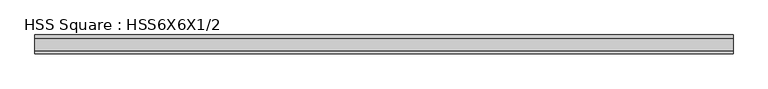
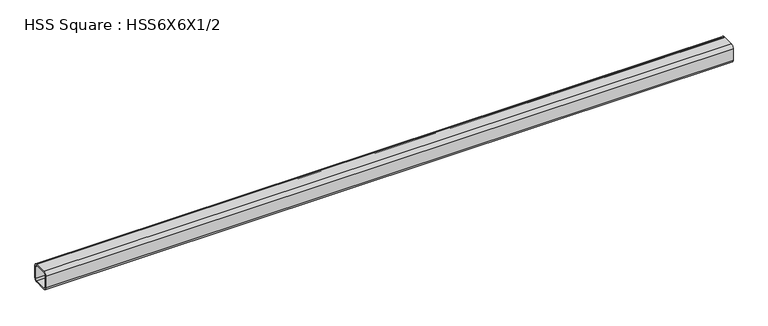
"""IFC4 building model written with IfcOpenShell, lengths in millimetres: member geometry, HSS Square : HSS6X6X1/2."""

from ifc_helpers import new_model, si_unit, point, frame, frame_2d, origin, place, context, project, spatial, polyline, circle_curve, trimmed, segment, composite_curve, outline, extrude, source, transform, mapped, element, save


def hss_square_hss6x6x1_2_6b3df641(model_context):
    return source(origin(), model_context, "Body", "SweptSolid", [
        extrude(outline(composite_curve([segment(polyline([(76.2, 50.8), (76.2, -50.8)]), True, "CONTINUOUS"), segment(trimmed(circle_curve(frame_2d((50.8, -50.8)), 25.4), [point((76.2, -50.8))], [point((50.8, -76.2))], False, "CARTESIAN"), True, "CONTINUOUS"), segment(polyline([(50.8, -76.2), (-50.8, -76.2)]), True, "CONTINUOUS"), segment(trimmed(circle_curve(frame_2d((-50.8, -50.8)), 25.4), [point((-50.8, -76.2))], [point((-76.2, -50.8))], False, "CARTESIAN"), True, "CONTINUOUS"), segment(polyline([(-76.2, -50.8), (-76.2, 50.8)]), True, "CONTINUOUS"), segment(trimmed(circle_curve(frame_2d((-50.8, 50.8)), 25.4), [point((-76.2, 50.8))], [point((-50.8, 76.2))], False, "CARTESIAN"), True, "CONTINUOUS"), segment(polyline([(-50.8, 76.2), (50.8, 76.2)]), True, "CONTINUOUS"), segment(trimmed(circle_curve(frame_2d((50.8, 50.8)), 25.4), [point((50.8, 76.2))], [point((76.2, 50.8))], False, "CARTESIAN"), True, "CONTINUOUS")], self_intersect=False), holes=[composite_curve([segment(trimmed(circle_curve(frame_2d((-50.8, 50.8)), 12.7), [point((-50.8, 63.5))], [point((-63.5, 50.8))], True, "CARTESIAN"), True, "CONTINUOUS"), segment(polyline([(-63.5, 50.8), (-63.5, -50.8)]), True, "CONTINUOUS"), segment(trimmed(circle_curve(frame_2d((-50.8, -50.8)), 12.7), [point((-63.5, -50.8))], [point((-50.8, -63.5))], True, "CARTESIAN"), True, "CONTINUOUS"), segment(polyline([(-50.8, -63.5), (50.8, -63.5)]), True, "CONTINUOUS"), segment(trimmed(circle_curve(frame_2d((50.8, -50.8)), 12.7), [point((50.8, -63.5))], [point((63.5, -50.8))], True, "CARTESIAN"), True, "CONTINUOUS"), segment(polyline([(63.5, -50.8), (63.5, 50.8)]), True, "CONTINUOUS"), segment(trimmed(circle_curve(frame_2d((50.8, 50.8)), 12.7), [point((63.5, 50.8))], [point((50.8, 63.5))], True, "CARTESIAN"), True, "CONTINUOUS"), segment(polyline([(50.8, 63.5), (-50.8, 63.5)]), True, "CONTINUOUS")], self_intersect=False)]), frame((-2805.6568492, 0.0, 0.0), z_axis=(1.0, 0.0, 0.0), x_axis=(0.0, 1.0, 0.0)), (0.0, 0.0, 1.0), 5611.3136984),
    ])


if __name__ == "__main__":
    model = new_model("IFC4")
    model_context = context("Model", 3, world=origin())
    ifc_project = project(units=[si_unit("LENGTHUNIT", "METRE", prefix="MILLI")], contexts=[model_context])
    site = spatial("IfcSite", under=ifc_project)
    building = spatial("IfcBuilding", under=site)
    placement = place(None, origin())
    hss_square_hss6x6x1_2_shape = hss_square_hss6x6x1_2_6b3df641(model_context)
    element("IfcMember", 1, ObjectType="HSS Square : HSS6X6X1/2", at=placement, inside=building, context=model_context, shape_type="MappedRepresentation", body=[
        mapped(hss_square_hss6x6x1_2_shape, transform((0.0, 0.0, 0.0), x_axis=(1.0, 0.0, 0.0), y_axis=(0.0, 1.0, 0.0), z_axis=(0.0, 0.0, 1.0))),
    ])
    save(model, "model.ifc")

# Revit data of these elements
# Type "HSS Square : HSS6X6X1/2"
#   Section Name Key = "HSS 6X6X1/2"
#   Assembly Code = "B10"
#   Width = 6.000"
#   Wall Nominal Thickness = 0.500"
#   Wall Design Thickness = 0.465"
#   Torsional Moment of Inertia = 81.10 in⁴
#   Torsional Modulus = 28.10 in³
#   Section Area = 9.74 in²
#   Plastic Modulus weak axis = 19.80 in³
#   Plastic Modulus strong axis = 19.80 in³
#   Outer Fillet = 1.000"
#   Nominal Weight = 35.24 lbf/ft
#   Moment of Inertia weak axis = 48.30 in⁴
#   Moment of Inertia strong axis = 48.30 in⁴
#   Inner Fillet = 0.500"
#   Height = 6.000"
#   Elastic Modulus weak axis = 16.10 in³
#   Elastic Modulus strong axis = 16.10 in³
#   Centroid Vertical = 3.000"
#   Centroid Horizontal = 3.000"
#   Length [instance default] = 5' - 0"
#   Structural Material [instance default] = Steel ASTM A500, Grade B, Rectangular and Square
#   Principal Axes Angle = 0
# Element 1 (IfcMember, "HSS Square : HSS6X6X1/2")
#   Structural Material = Steel ASTM A36
#   Materials on its faces: "Steel ASTM A36"
# Materials
#   "Steel ASTM A500, Grade B, Rectangular and Square": class "Metal", colour RGB 199 199 199, transparency 0, Description = "Carbon steel", Cost = 0
#   "Steel ASTM A36": class "Metal", colour RGB 199 199 199, transparency 0, Description = "Structural steel, ASTM A36 Grade B, mill finish", Cost = 0
